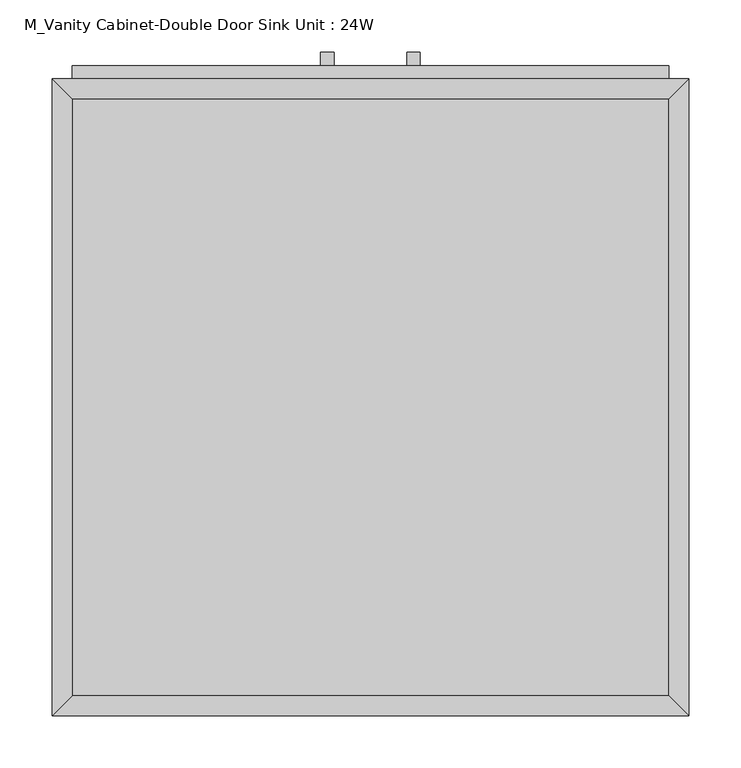
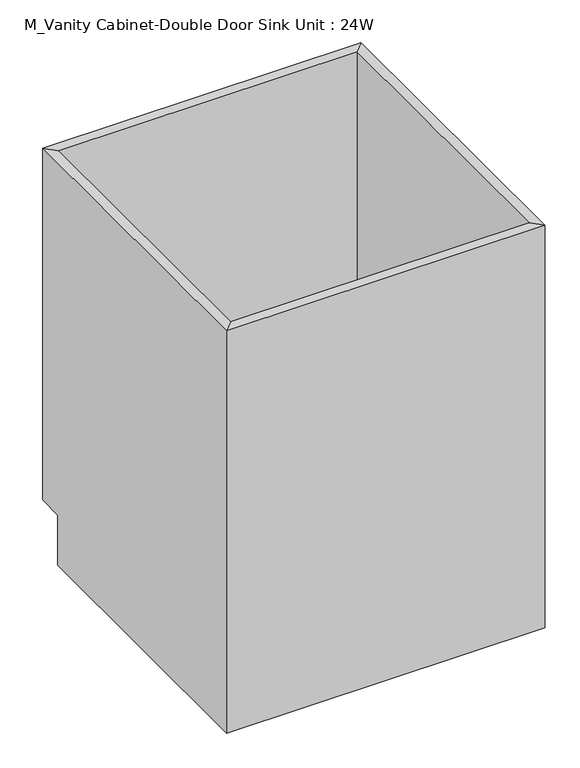
"""IFC4 building model written with IfcOpenShell, lengths in millimetres: furniture geometry, M_Vanity Cabinet-Double Door Sink Unit : 24W."""

from ifc_helpers import new_model, si_unit, frame, origin, place, context, project, spatial, polyline, outline, extrude, faceted_brep, source, transform, mapped, element, save


def m_vanity_cabinet_double_door_sink_unit_24w_43da309b(model_context):
    return source(origin(), model_context, "Body", "SolidModel", [
        faceted_brep([(304.4877049, 590.55, 812.8), (-267.0122951, 590.55, 812.8), (-267.0122951, 590.55, 101.6), (304.4877049, 590.55, 101.6), (323.5377049, 609.6, 812.8), (-286.0622951, 609.6, 812.8), (323.5377049, 609.6, 101.6), (-286.0622951, 609.6, 101.6), (-267.0122951, 19.05, 812.8), (-267.0122951, 19.05, 101.6), (-267.0122951, 558.8, 101.6), (-286.0622951, 0.0, 812.8), (-286.0622951, 558.8, 101.6), (-286.0622951, 558.8, 0.0), (-286.0622951, 0.0, 0.0), (304.4877049, 19.05, 812.8), (304.4877049, 19.05, 101.6), (323.5377049, 0.0, 812.8), (323.5377049, 0.0, 0.0), (304.4877049, 558.8, 101.6), (323.5377049, 558.8, 0.0), (323.5377049, 558.8, 101.6)], [[[0, 1, 2, 3]], [[0, 4, 5, 1]], [[4, 6, 7, 5]], [[2, 7, 6, 3]], [[1, 8, 9, 10, 2]], [[5, 11, 8, 1]], [[7, 12, 13, 14, 11, 5]], [[2, 10, 12, 7]], [[8, 15, 16, 9]], [[11, 17, 15, 8]], [[14, 18, 17, 11]], [[3, 19, 16, 15, 0]], [[0, 15, 17, 4]], [[4, 17, 18, 20, 21, 6]], [[6, 21, 19, 3]], [[10, 9, 16, 19]], [[18, 14, 13, 20]], [[13, 12, 10, 19, 21, 20]]]),
        extrude(outline(polyline([(-16.1872951, 635.0), (-16.1872951, 622.3), (-28.8872951, 622.3), (-28.8872951, 635.0), (-16.1872951, 635.0)])), frame((0.0, 0.0, 510.269895), z_axis=(0.0, 0.0, 1.0), x_axis=(1.0, 0.0, 0.0)), (0.0, 0.0, 1.0), 124.730105),
        extrude(outline(polyline([(66.3627049, 635.0), (66.3627049, 622.3), (53.6627049, 622.3), (53.6627049, 635.0), (66.3627049, 635.0)])), frame((0.0, 0.0, 510.269895), z_axis=(0.0, 0.0, 1.0), x_axis=(1.0, 0.0, 0.0)), (0.0, 0.0, 1.0), 124.730105),
        extrude(outline(polyline([(9.2127049, 622.3), (9.2127049, 609.6), (-267.0122951, 609.6), (-267.0122951, 622.3), (9.2127049, 622.3)])), frame((0.0, 0.0, 120.65), z_axis=(0.0, 0.0, 1.0), x_axis=(1.0, 0.0, 0.0)), (0.0, 0.0, 1.0), 552.45),
        extrude(outline(polyline([(304.4877049, 622.3), (304.4877049, 609.6), (28.2627049, 609.6), (28.2627049, 622.3), (304.4877049, 622.3)])), frame((0.0, 0.0, 120.65), z_axis=(0.0, 0.0, 1.0), x_axis=(1.0, 0.0, 0.0)), (0.0, 0.0, 1.0), 552.45),
        extrude(outline(polyline([(304.4877049, 622.3), (304.4877049, 609.6), (-267.0122951, 609.6), (-267.0122951, 622.3), (304.4877049, 622.3)])), frame((0.0, 0.0, 692.15), z_axis=(0.0, 0.0, 1.0), x_axis=(1.0, 0.0, 0.0)), (0.0, 0.0, 1.0), 101.6),
        extrude(outline(polyline([(304.4877049, 19.05), (-267.0122951, 19.05), (-267.0122951, 590.55), (304.4877049, 590.55), (304.4877049, 19.05)])), frame((0.0, 0.0, 101.6), z_axis=(0.0, 0.0, 1.0), x_axis=(1.0, 0.0, 0.0)), (0.0, 0.0, 1.0), 19.05),
    ])


if __name__ == "__main__":
    model = new_model("IFC4")
    model_context = context("Model", 3, world=origin())
    ifc_project = project(units=[si_unit("LENGTHUNIT", "METRE", prefix="MILLI")], contexts=[model_context])
    site = spatial("IfcSite", under=ifc_project)
    building = spatial("IfcBuilding", under=site)
    placement = place(None, origin())
    m_vanity_cabinet_double_door_sink_unit_24w_shape = m_vanity_cabinet_double_door_sink_unit_24w_43da309b(model_context)
    element("IfcFurniture", 1, ObjectType="M_Vanity Cabinet-Double Door Sink Unit : 24W", at=placement, inside=building, context=model_context, shape_type="MappedRepresentation", body=[
        mapped(m_vanity_cabinet_double_door_sink_unit_24w_shape, transform((0.0, 0.0, 0.0), x_axis=(1.0, 0.0, 0.0), y_axis=(0.0, 1.0, 0.0), z_axis=(0.0, 0.0, 1.0))),
    ])
    save(model, "model.ifc")

# Revit data of these elements
# Type "M_Vanity Cabinet-Double Door Sink Unit : 24W"
#   Depth = 2' - 0"
#   Height = 2' - 8"
#   Plinth Depth = 0' - 2"
#   Plinth Height = 0' - 4"
#   Width = 2' - 0"
#   Cabinet Material = none
#   Door/Drawer Material = none
#   Handle Material = Cabinets - Handles
# Element 1 (IfcFurniture, "M_Vanity Cabinet-Double Door Sink Unit : 24W")
#   Materials on its faces: "MAX HEIGHT OF  COUNTERTOP 34\"", "Cabinets - Handles"
# Materials
#   "Cabinets - Handles": class "Metal", colour RGB 57 57 57, transparency 0
#   "MAX HEIGHT OF  COUNTERTOP 34\"": class "Generic", colour RGB 181 181 181, transparency 0, Cost = 0
